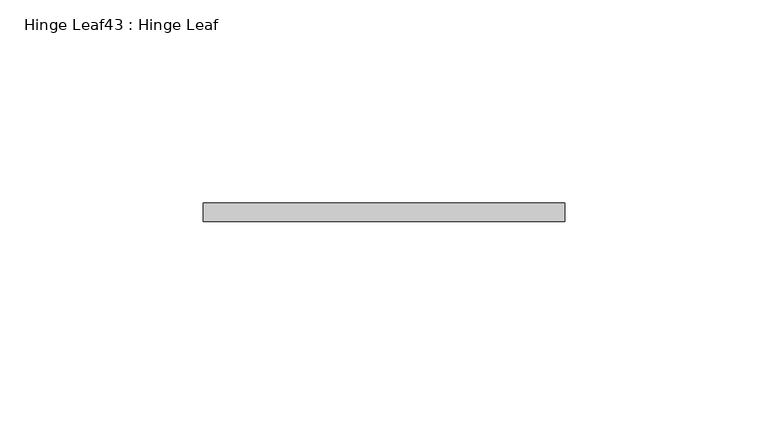
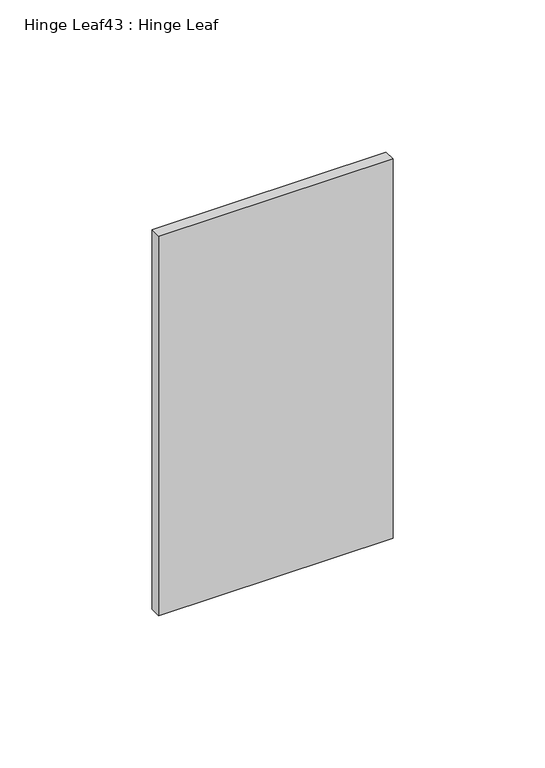
"""IFC4 building model written with IfcOpenShell, lengths in millimetres: proxy geometry, Hinge Leaf43 : Hinge Leaf."""

from ifc_helpers import new_model, si_unit, frame, origin, place, context, project, spatial, polyline, outline, extrude, source, transform, mapped, element, save


def hinge_leaf43_hinge_leaf_a46fc4d1(model_context):
    return source(origin(), model_context, "Body", "SweptSolid", [
        extrude(outline(polyline([(587327.7934739, -534096.6663841), (587416.6934739, -534096.6663841), (587416.6934739, -534101.2383841), (587327.7934739, -534101.2383841), (587327.7934739, -534096.6663841)])), frame((0.0, 0.0, 1123.95), z_axis=(0.0, 0.0, 1.0), x_axis=(1.0, 0.0, 0.0)), (0.0, 0.0, 1.0), 152.4),
    ])


if __name__ == "__main__":
    model = new_model("IFC4")
    model_context = context("Model", 3, world=origin())
    ifc_project = project(units=[si_unit("LENGTHUNIT", "METRE", prefix="MILLI")], contexts=[model_context])
    site = spatial("IfcSite", under=ifc_project)
    building = spatial("IfcBuilding", under=site)
    placement = place(None, origin())
    hinge_leaf43_hinge_leaf_shape = hinge_leaf43_hinge_leaf_a46fc4d1(model_context)
    element("IfcBuildingElementProxy", 1, Name="Hinge Leaf43 : Hinge Leaf", ObjectType="Hinge Leaf43 : Hinge Leaf", at=placement, inside=building, context=model_context, shape_type="MappedRepresentation", body=[
        mapped(hinge_leaf43_hinge_leaf_shape, transform((0.0, 0.0, 0.0), x_axis=(1.0, 0.0, 0.0), y_axis=(0.0, 1.0, 0.0), z_axis=(0.0, 0.0, 1.0))),
    ])
    save(model, "model.ifc")

# Revit data of these elements
# Element 1 (IfcBuildingElementProxy, "Hinge Leaf43 : Hinge Leaf")
#   Materials on its faces: "6\"X6\" WELD-ON STL BUTT HINGE"
# Materials
#   "6\"X6\" WELD-ON STL BUTT HINGE": class "Metal", colour RGB 189 187 185, transparency 0, Description = "Carbon steel", Cost = 0
